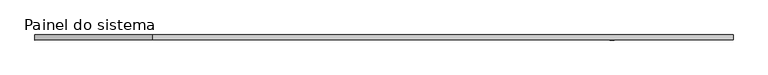
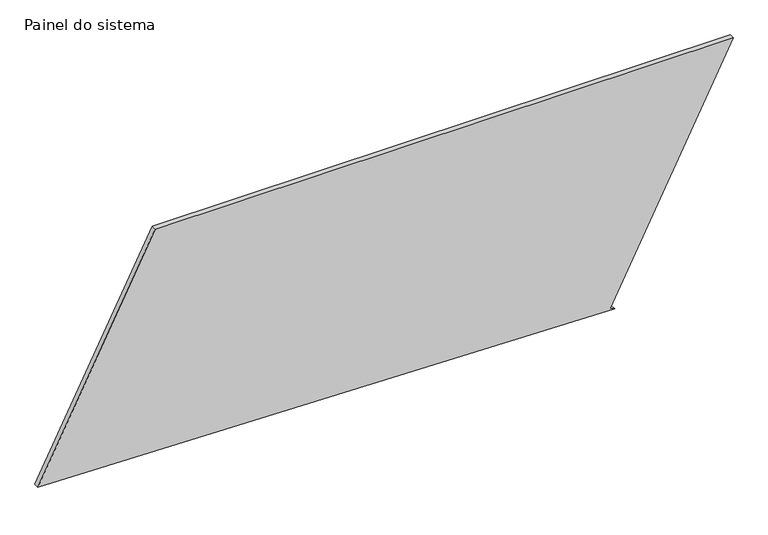
"""IFC4 building model written with IfcOpenShell, lengths in millimetres: plate geometry, Painel do sistema : Envidraçado."""

from ifc_helpers import new_model, si_unit, frame, origin, place, context, project, spatial, polyline, outline, extrude, source, transform, mapped, element, save


def painel_do_sistema_e6994196(model_context):
    return source(origin(), model_context, "Body", "SweptSolid", [
        extrude(outline(polyline([(0.0, 1132.38167), (11.291819, 1110.077078), (1211.249627, 1717.5621342), (1211.249627, -1137.9361331), (66.32147, -1717.5621342), (0.0, 1132.38167)])), frame((0.0, 24.5, 0.0), z_axis=(0.0, 1.0, 0.0), x_axis=(0.0, 0.0, 1.0)), (0.0, 0.0, 1.0), 25.0),
    ])


if __name__ == "__main__":
    model = new_model("IFC4")
    model_context = context("Model", 3, world=origin())
    ifc_project = project(units=[si_unit("LENGTHUNIT", "METRE", prefix="MILLI")], contexts=[model_context])
    site = spatial("IfcSite", under=ifc_project)
    building = spatial("IfcBuilding", under=site)
    placement = place(None, origin())
    painel_do_sistema_shape = painel_do_sistema_e6994196(model_context)
    element("IfcPlate", 1, ObjectType="Painel do sistema : Envidraçado", at=placement, inside=building, context=model_context, shape_type="MappedRepresentation", body=[
        mapped(painel_do_sistema_shape, transform((0.0, 0.0, 0.0), x_axis=(1.0, 0.0, 0.0), y_axis=(0.0, 1.0, 0.0), z_axis=(0.0, 0.0, 1.0))),
    ])
    save(model, "model.ifc")

# Revit data of these elements
# Type "Painel do sistema : Envidraçado"
#   Construction Type Id = "GSP4R"
#   Analytic Construction = "Vidraça única Pilkington 1/8 pol"
#   Visual Light Transmittance = 0.9
#   Solar Heat Gain Coefficient = 0.86
#   Heat Transfer Coefficient (U) = 6.7069 W/(m²·K)
# Element 1 (IfcPlate, "Painel do sistema : Envidraçado")
#   Materials on its faces: "Vidro"
# Materials
#   "Vidro": class "Vidro", colour RGB 0 128 192, transparency 0.9, Description = "Vidro de sílica", Cost = 0
